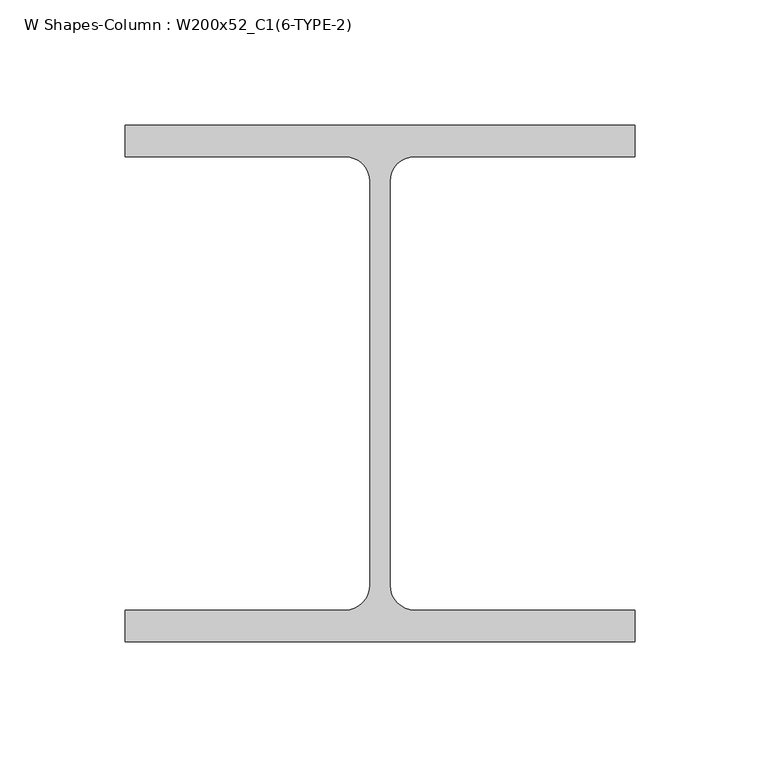
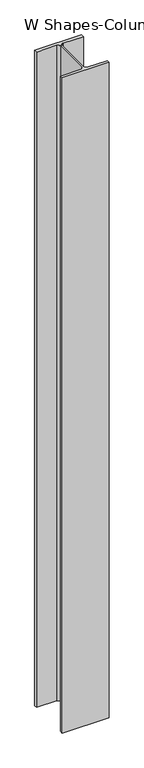
"""IFC4 building model written with IfcOpenShell, lengths in millimetres: column geometry, W Shapes-Column : W200x52_C1(6-TYPE-2)."""

import ifcopenshell
import ifcopenshell.guid

model = None  # the IFC model being written
_history = None  # IfcOwnerHistory: only IFC2X3 demands one
_inside = {}  # id of a spatial element -> (the spatial element, [elements in it])
_under = {}  # id of a project, library or spatial element -> (it, [spatial elements below it])
_declared = {}  # id of a project -> (the project, [libraries it declares])
_typed = {}  # id of a type object -> (the type object, [elements of that type])
_made_of = {}  # id of a material, layer set ... -> (it, [elements and type objects made of it])


def new_model(schema):
    """Start an empty IFC model of exactly this schema.

    Asked for "IFC4X3", IfcOpenShell would pick the latest addendum, in which some entities
    have other attributes; the version numbers below select the first issue.
    IFC2X3 requires an IfcOwnerHistory on every rooted entity: one is made here for all.
    """
    global model, _history
    if schema == "IFC4X3":
        model = ifcopenshell.file(schema_version=(4, 3, 0, 0))
    else:
        model = ifcopenshell.file(schema=schema)
    _inside.clear()
    _under.clear()
    _declared.clear()
    _typed.clear()
    _made_of.clear()
    _history = None
    if model.schema == "IFC2X3":
        org = make("IfcOrganization", Name="unknown")
        user = make(
            "IfcPersonAndOrganization",
            ThePerson=make("IfcPerson", FamilyName="unknown"),
            TheOrganization=org,
        )
        app = make(
            "IfcApplication",
            ApplicationDeveloper=org,
            Version="unknown",
            ApplicationFullName="unknown",
            ApplicationIdentifier="unknown",
        )
        _history = make(
            "IfcOwnerHistory",
            OwningUser=user,
            OwningApplication=app,
            ChangeAction="ADDED",
            CreationDate=0,
        )
    return model


def make(cls, **values):
    """One entity of the class cls with the attributes given. An attribute that is None is left unset."""
    return model.create_entity(
        cls, **{name: value for name, value in values.items() if value is not None}
    )


def rooted(cls, **values):
    """An entity with a GlobalId (a new one), such as an element, a storey or a relation."""
    return make(cls, GlobalId=ifcopenshell.guid.new(), OwnerHistory=_history, **values)


def si_unit(unit_type, name, prefix=None):
    """IfcSIUnit, for example si_unit("LENGTHUNIT", "METRE", prefix="MILLI")."""
    return make("IfcSIUnit", UnitType=unit_type, Prefix=prefix, Name=name)


def assignment(units):
    """IfcUnitAssignment: the units of a project."""
    return None if units is None else make("IfcUnitAssignment", Units=units)


def point(xyz):
    """IfcCartesianPoint."""
    return None if xyz is None else make("IfcCartesianPoint", Coordinates=xyz)


def direction(xyz):
    """IfcDirection."""
    return None if xyz is None else make("IfcDirection", DirectionRatios=xyz)


def frame(location, z_axis=None, x_axis=None):
    """IfcAxis2Placement3D, a coordinate frame: its origin and axes. An axis left out is left unset."""
    return make(
        "IfcAxis2Placement3D",
        Location=point(location),
        Axis=direction(z_axis),
        RefDirection=direction(x_axis),
    )


def frame_2d(location, x_axis=None):
    """IfcAxis2Placement2D, a coordinate frame in the plane: its origin and x axis."""
    return make(
        "IfcAxis2Placement2D", Location=point(location), RefDirection=direction(x_axis)
    )


def origin():
    """The frame at (0, 0, 0) with its axes left unset."""
    return frame((0.0, 0.0, 0.0))


def place(relative_to, where):
    """IfcLocalPlacement: puts the frame where relative to a parent placement (None: the world)."""
    return make(
        "IfcLocalPlacement", PlacementRelTo=relative_to, RelativePlacement=where
    )


def context(
    kind, dimensions, precision=None, world=None, true_north=None, identifier=None
):
    """IfcGeometricRepresentationContext, for example the 3D "Model" context."""
    return make(
        "IfcGeometricRepresentationContext",
        ContextIdentifier=identifier,
        ContextType=kind,
        CoordinateSpaceDimension=dimensions,
        Precision=precision,
        WorldCoordinateSystem=world,
        TrueNorth=true_north,
    )


def project(units=None, contexts=None):
    """IfcProject with its units and contexts."""
    return rooted(
        "IfcProject",
        Name="project",
        RepresentationContexts=contexts,
        UnitsInContext=assignment(units),
    )


def spatial(cls, under=None, at=None, **own):
    """A site, building, storey or space (cls), placed at a placement, below another one or the project."""
    s = rooted(cls, ObjectPlacement=at, **own)
    if under is not None:
        _under.setdefault(under.id(), (under, []))[1].append(s)
    return s


def polyline(points):
    """IfcPolyline through the points."""
    return make("IfcPolyline", Points=[point(p) for p in points])


def circle_curve(where, radius):
    """IfcCircle in the frame where."""
    return make("IfcCircle", Position=where, Radius=radius)


def trimmed(basis, trim1, trim2, sense, master):
    """IfcTrimmedCurve: the piece of a basis curve between two trims."""
    return make(
        "IfcTrimmedCurve",
        BasisCurve=basis,
        Trim1=trim1,
        Trim2=trim2,
        SenseAgreement=sense,
        MasterRepresentation=master,
    )


def segment(curve, same_sense, transition):
    """IfcCompositeCurveSegment."""
    return make(
        "IfcCompositeCurveSegment",
        Transition=transition,
        SameSense=same_sense,
        ParentCurve=curve,
    )


def composite_curve(segments, self_intersect=None):
    """IfcCompositeCurve: segments joined end to end."""
    return make("IfcCompositeCurve", Segments=segments, SelfIntersect=self_intersect)


def outline(outer, holes=None, kind="AREA"):
    """IfcArbitraryClosedProfileDef: a profile drawn as a closed curve; with holes, ...WithVoids."""
    if holes is None:
        return make("IfcArbitraryClosedProfileDef", ProfileType=kind, OuterCurve=outer)
    return make(
        "IfcArbitraryProfileDefWithVoids",
        ProfileType=kind,
        OuterCurve=outer,
        InnerCurves=holes,
    )


def extrude(swept, where, along, depth):
    """IfcExtrudedAreaSolid: the profile swept, set in the frame where, extruded along a direction by depth."""
    return make(
        "IfcExtrudedAreaSolid",
        SweptArea=swept,
        Position=where,
        ExtrudedDirection=direction(along),
        Depth=depth,
    )


def shape(context_of_items, identifier, shape_type, items):
    """IfcShapeRepresentation: the items that make up one representation, for example the "Body"."""
    return make(
        "IfcShapeRepresentation",
        ContextOfItems=context_of_items,
        RepresentationIdentifier=identifier,
        RepresentationType=shape_type,
        Items=items,
    )


def source(mapping_origin, context_of_items, identifier, shape_type, items):
    """IfcRepresentationMap: a shape defined once, which mapped items show again and again."""
    return make(
        "IfcRepresentationMap",
        MappingOrigin=mapping_origin,
        MappedRepresentation=shape(context_of_items, identifier, shape_type, items),
    )


def transform(
    local_origin,
    x_axis=None,
    y_axis=None,
    z_axis=None,
    scale=None,
    scale2=None,
    scale3=None,
    uniform=True,
):
    """IfcCartesianTransformationOperator3D, or its non-uniform kind. x_axis, y_axis, z_axis: its Axis1, 2, 3."""
    if uniform:
        return make(
            "IfcCartesianTransformationOperator3D",
            Axis1=direction(x_axis),
            Axis2=direction(y_axis),
            LocalOrigin=point(local_origin),
            Scale=scale,
            Axis3=direction(z_axis),
        )
    return make(
        "IfcCartesianTransformationOperator3DnonUniform",
        Axis1=direction(x_axis),
        Axis2=direction(y_axis),
        LocalOrigin=point(local_origin),
        Scale=scale,
        Axis3=direction(z_axis),
        Scale2=scale2,
        Scale3=scale3,
    )


def mapped(mapping_source, mapping_target):
    """IfcMappedItem: shows the shape of a source again, moved by a transform."""
    return make(
        "IfcMappedItem", MappingSource=mapping_source, MappingTarget=mapping_target
    )


def made_of(thing, what):
    """Note that an element or type object is made of a material, layer set ...; save() writes the relation."""
    if what is not None:
        _made_of.setdefault(what.id(), (what, []))[1].append(thing)
    return thing


def element(
    cls,
    number,
    at=None,
    inside=None,
    cuts=None,
    type_object=None,
    material=None,
    context=None,
    identifier="Body",
    shape_type=None,
    held_by="IfcProductDefinitionShape",
    body=None,
    shapes=None,
    **own,
):
    """One element of the class cls, such as IfcWall. Its Tag is "e" and its number.

    at: its placement. inside: the storey or other place that contains it. cuts: it is an
    opening in that element (IfcRelVoidsElement). A single representation is given by context,
    identifier, shape_type and body (its items); several are given by shapes. held_by: the class
    of the entity that holds the representations. save() writes the other relations.
    """
    e = rooted(cls, Tag="e%d" % number, ObjectPlacement=at, **own)
    if body is not None:
        shapes = [shape(context, identifier, shape_type, body)]
    if shapes is not None:
        e.Representation = make(held_by, Representations=shapes)
    if inside is not None:
        _inside.setdefault(inside.id(), (inside, []))[1].append(e)
    if cuts is not None:
        rooted(
            "IfcRelVoidsElement", RelatingBuildingElement=cuts, RelatedOpeningElement=e
        )
    if type_object is not None:
        _typed.setdefault(type_object.id(), (type_object, []))[1].append(e)
    return made_of(e, material)


def aggregate(whole, parts):
    """IfcRelAggregates: a whole, such as a stair, and the parts it consists of."""
    return rooted("IfcRelAggregates", RelatingObject=whole, RelatedObjects=parts)


def save(model, path):
    """Write the relations noted so far, then the file.

    IfcRelAggregates (storeys below a building ...), IfcRelContainedInSpatialStructure (elements
    in a storey), IfcRelDefinesByType, IfcRelAssociatesMaterial and IfcRelDeclares: one each for
    every whole, place, type object, material and project.
    """
    for whole, parts in _under.values():
        aggregate(whole, parts)
    for where, things in _inside.values():
        rooted(
            "IfcRelContainedInSpatialStructure",
            RelatedElements=things,
            RelatingStructure=where,
        )
    for kind, things in _typed.values():
        rooted("IfcRelDefinesByType", RelatedObjects=things, RelatingType=kind)
    for what, things in _made_of.values():
        rooted("IfcRelAssociatesMaterial", RelatedObjects=things, RelatingMaterial=what)
    for by, libraries in _declared.values():
        rooted("IfcRelDeclares", RelatingContext=by, RelatedDefinitions=libraries)
    model.write(path)


def w_shapes_column_w200x52_c1_6_type_2_262f380d(model_context):
    return source(origin(), model_context, "Body", "SweptSolid", [
        extrude(outline(composite_curve([segment(polyline([(101.854, -103.124), (-101.854, -103.124), (-101.854, -90.551), (-13.9446, -90.551)]), True, "CONTINUOUS"), segment(trimmed(circle_curve(frame_2d((-13.9446, -80.5434)), 10.0076), [point((-13.9446, -90.551))], [point((-3.937, -80.5434))], True, "CARTESIAN"), True, "CONTINUOUS"), segment(polyline([(-3.937, -80.5434), (-3.937, 80.5434)]), True, "CONTINUOUS"), segment(trimmed(circle_curve(frame_2d((-13.9446, 80.5434)), 10.0076), [point((-3.937, 80.5434))], [point((-13.9446, 90.551))], True, "CARTESIAN"), True, "CONTINUOUS"), segment(polyline([(-13.9446, 90.551), (-101.854, 90.551), (-101.854, 103.124), (101.854, 103.124), (101.854, 90.551), (13.9446, 90.551)]), True, "CONTINUOUS"), segment(trimmed(circle_curve(frame_2d((13.9446, 80.5434)), 10.0076), [point((13.9446, 90.551))], [point((3.937, 80.5434))], True, "CARTESIAN"), True, "CONTINUOUS"), segment(polyline([(3.937, 80.5434), (3.937, -80.5434)]), True, "CONTINUOUS"), segment(trimmed(circle_curve(frame_2d((13.9446, -80.5434)), 10.0076), [point((3.937, -80.5434))], [point((13.9446, -90.551))], True, "CARTESIAN"), True, "CONTINUOUS"), segment(polyline([(13.9446, -90.551), (101.854, -90.551), (101.854, -103.124)]), True, "CONTINUOUS")], self_intersect=False)), frame((0.0, 0.0, 9260.0), z_axis=(0.0, 0.0, 1.0), x_axis=(1.0, 0.0, 0.0)), (0.0, 0.0, 1.0), 3000.0),
    ])


if __name__ == "__main__":
    model = new_model("IFC4")
    model_context = context("Model", 3, world=origin())
    ifc_project = project(units=[si_unit("LENGTHUNIT", "METRE", prefix="MILLI")], contexts=[model_context])
    site = spatial("IfcSite", under=ifc_project)
    building = spatial("IfcBuilding", under=site)
    placement = place(None, origin())
    w_shapes_column_w200x52_c1_6_type_2_shape = w_shapes_column_w200x52_c1_6_type_2_262f380d(model_context)
    element("IfcColumn", 1, ObjectType="W Shapes-Column : W200x52_C1(6-TYPE-2)", at=placement, inside=building, context=model_context, shape_type="MappedRepresentation", body=[
        mapped(w_shapes_column_w200x52_c1_6_type_2_shape, transform((0.0, 0.0, 0.0), x_axis=(1.0, 0.0, 0.0), y_axis=(0.0, 1.0, 0.0), z_axis=(0.0, 0.0, 1.0))),
    ])
    save(model, "model.ifc")

# Revit data of these elements
# Type "W Shapes-Column : W200x52_C1(6-TYPE-2)"
#   Section Name Key = "W8X35"
#   Assembly Code = "B10"
#   Width = 20.3708 cm
#   Web Thickness = 0.7874 cm
#   Web Fillet = 1.0008 cm
#   Warping Constant = 166223.7 cm⁶
#   Torsional Moment of Inertia = 32.0082 cm⁴
#   Section Area = 66.4515 cm²
#   Plastic Modulus weak axis = 263.832 cm³
#   Plastic Modulus strong axis = 568.631 cm³
#   Perimeter = 1.1936 m²/m
#   Nominal Weight = 52.0857 kgf/m
#   Moment of Inertia weak axis = 1773.15 cm⁴
#   Moment of Inertia strong axis = 5286.14 cm⁴
#   Height = 20.6248 cm
#   Flange Thickness = 1.2573 cm
#   Elastic Modulus weak axis = 173.703 cm³
#   Elastic Modulus strong axis = 511.276 cm³
#   Clear Web Height = 14.605 cm
#   Centroid Vertical = 10.3124 cm
#   Centroid Horizontal = 10.1854 cm
#   Bolt Spacing = 13.97 cm
#   Structural Material [instance default] = Steel ASTM A992
#   Principal Axes Angle = 0
# Element 1 (IfcColumn, "W Shapes-Column : W200x52_C1(6-TYPE-2)")
#   Structural Material = none
# Materials
#   "Steel ASTM A992": class "Metal", colour RGB 199 199 199, transparency 0, Description = "Structural steel 50ksi", Cost = 0
